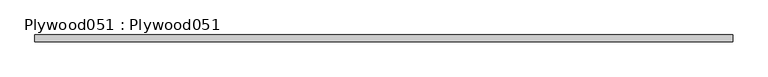
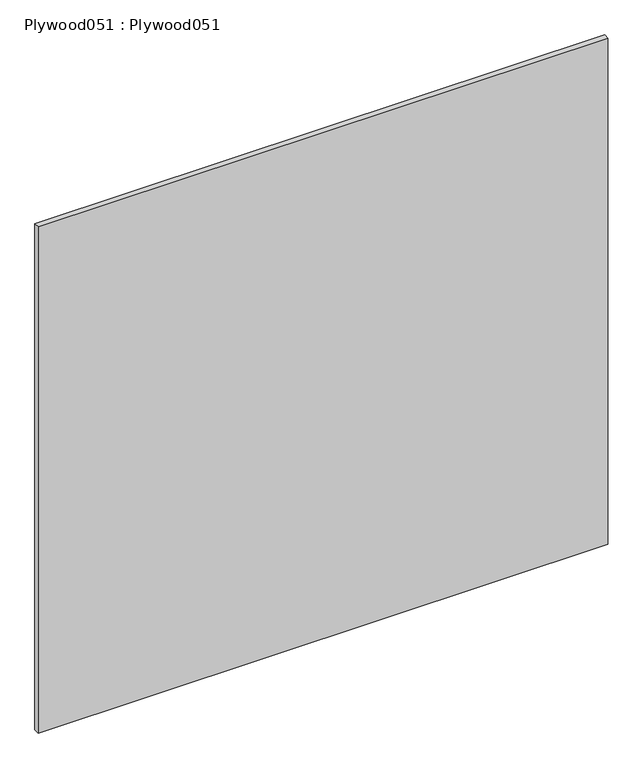
"""IFC4 building model written with IfcOpenShell, lengths in millimetres: proxy geometry, Plywood051 : Plywood051."""

from ifc_helpers import new_model, si_unit, frame, origin, place, context, project, spatial, polyline, outline, extrude, source, transform, mapped, element, save


def plywood051_plywood051_f8ddbb65(model_context):
    return source(origin(), model_context, "Body", "SweptSolid", [
        extrude(outline(polyline([(14383.0178845, -4637.5425368), (14383.0178845, -4656.5894118), (12383.0178845, -4656.5894118), (12383.0178845, -4637.5425368), (14383.0178845, -4637.5425368)])), frame((0.0, 0.0, 36531.296), z_axis=(0.0, 0.0, 1.0), x_axis=(1.0, 0.0, 0.0)), (0.0, 0.0, 1.0), 1879.6),
    ])


if __name__ == "__main__":
    model = new_model("IFC4")
    model_context = context("Model", 3, world=origin())
    ifc_project = project(units=[si_unit("LENGTHUNIT", "METRE", prefix="MILLI")], contexts=[model_context])
    site = spatial("IfcSite", under=ifc_project)
    building = spatial("IfcBuilding", under=site)
    placement = place(None, origin())
    plywood051_plywood051_shape = plywood051_plywood051_f8ddbb65(model_context)
    element("IfcBuildingElementProxy", 1, Name="Plywood051 : Plywood051", ObjectType="Plywood051 : Plywood051", at=placement, inside=building, context=model_context, shape_type="MappedRepresentation", body=[
        mapped(plywood051_plywood051_shape, transform((0.0, 0.0, 0.0), x_axis=(1.0, 0.0, 0.0), y_axis=(0.0, 1.0, 0.0), z_axis=(0.0, 0.0, 1.0))),
    ])
    save(model, "model.ifc")

# Revit data of these elements
# Type "Plywood051 : Plywood051"
#   NameOverride = "Plywood051"
# Element 1 (IfcBuildingElementProxy, "Plywood051 : Plywood051")
#   Materials on its faces: "CDX PLYWOOD - SEE STRUCTURAL DWGS"
# Materials
#   "CDX PLYWOOD - SEE STRUCTURAL DWGS": class "Unassigned", colour RGB 177 130 114, transparency 0, Cost = 0
